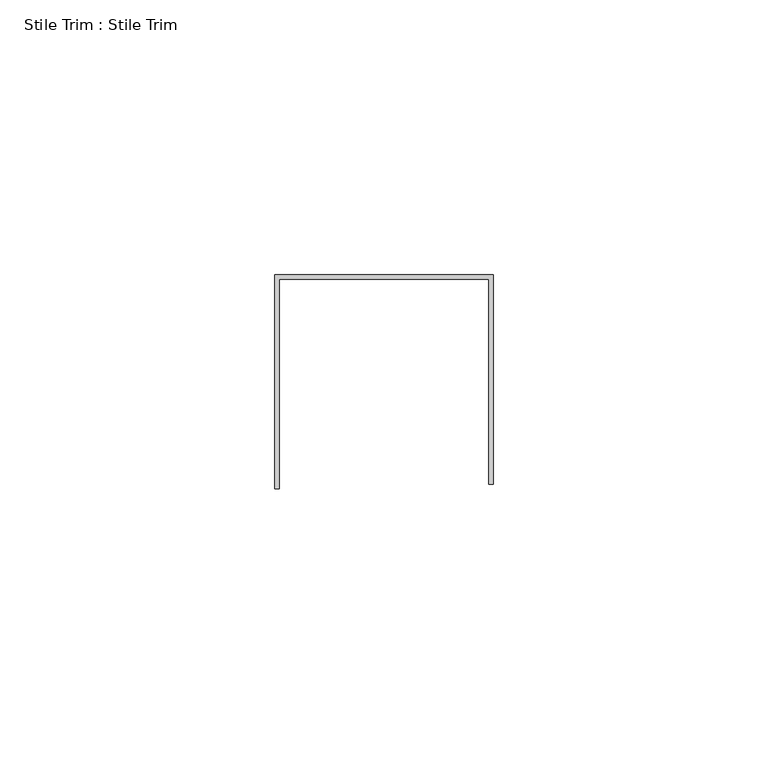
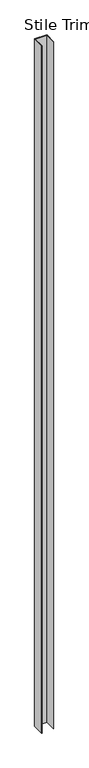
"""IFC4 building model written with IfcOpenShell, lengths in millimetres: proxy geometry, Stile Trim : Stile Trim."""

import ifcopenshell
import ifcopenshell.guid

model = None  # the IFC model being written
_history = None  # IfcOwnerHistory: only IFC2X3 demands one
_inside = {}  # id of a spatial element -> (the spatial element, [elements in it])
_under = {}  # id of a project, library or spatial element -> (it, [spatial elements below it])
_declared = {}  # id of a project -> (the project, [libraries it declares])
_typed = {}  # id of a type object -> (the type object, [elements of that type])
_made_of = {}  # id of a material, layer set ... -> (it, [elements and type objects made of it])


def new_model(schema):
    """Start an empty IFC model of exactly this schema.

    Asked for "IFC4X3", IfcOpenShell would pick the latest addendum, in which some entities
    have other attributes; the version numbers below select the first issue.
    IFC2X3 requires an IfcOwnerHistory on every rooted entity: one is made here for all.
    """
    global model, _history
    if schema == "IFC4X3":
        model = ifcopenshell.file(schema_version=(4, 3, 0, 0))
    else:
        model = ifcopenshell.file(schema=schema)
    _inside.clear()
    _under.clear()
    _declared.clear()
    _typed.clear()
    _made_of.clear()
    _history = None
    if model.schema == "IFC2X3":
        org = make("IfcOrganization", Name="unknown")
        user = make(
            "IfcPersonAndOrganization",
            ThePerson=make("IfcPerson", FamilyName="unknown"),
            TheOrganization=org,
        )
        app = make(
            "IfcApplication",
            ApplicationDeveloper=org,
            Version="unknown",
            ApplicationFullName="unknown",
            ApplicationIdentifier="unknown",
        )
        _history = make(
            "IfcOwnerHistory",
            OwningUser=user,
            OwningApplication=app,
            ChangeAction="ADDED",
            CreationDate=0,
        )
    return model


def make(cls, **values):
    """One entity of the class cls with the attributes given. An attribute that is None is left unset."""
    return model.create_entity(
        cls, **{name: value for name, value in values.items() if value is not None}
    )


def rooted(cls, **values):
    """An entity with a GlobalId (a new one), such as an element, a storey or a relation."""
    return make(cls, GlobalId=ifcopenshell.guid.new(), OwnerHistory=_history, **values)


def si_unit(unit_type, name, prefix=None):
    """IfcSIUnit, for example si_unit("LENGTHUNIT", "METRE", prefix="MILLI")."""
    return make("IfcSIUnit", UnitType=unit_type, Prefix=prefix, Name=name)


def assignment(units):
    """IfcUnitAssignment: the units of a project."""
    return None if units is None else make("IfcUnitAssignment", Units=units)


def point(xyz):
    """IfcCartesianPoint."""
    return None if xyz is None else make("IfcCartesianPoint", Coordinates=xyz)


def direction(xyz):
    """IfcDirection."""
    return None if xyz is None else make("IfcDirection", DirectionRatios=xyz)


def frame(location, z_axis=None, x_axis=None):
    """IfcAxis2Placement3D, a coordinate frame: its origin and axes. An axis left out is left unset."""
    return make(
        "IfcAxis2Placement3D",
        Location=point(location),
        Axis=direction(z_axis),
        RefDirection=direction(x_axis),
    )


def origin():
    """The frame at (0, 0, 0) with its axes left unset."""
    return frame((0.0, 0.0, 0.0))


def place(relative_to, where):
    """IfcLocalPlacement: puts the frame where relative to a parent placement (None: the world)."""
    return make(
        "IfcLocalPlacement", PlacementRelTo=relative_to, RelativePlacement=where
    )


def context(
    kind, dimensions, precision=None, world=None, true_north=None, identifier=None
):
    """IfcGeometricRepresentationContext, for example the 3D "Model" context."""
    return make(
        "IfcGeometricRepresentationContext",
        ContextIdentifier=identifier,
        ContextType=kind,
        CoordinateSpaceDimension=dimensions,
        Precision=precision,
        WorldCoordinateSystem=world,
        TrueNorth=true_north,
    )


def project(units=None, contexts=None):
    """IfcProject with its units and contexts."""
    return rooted(
        "IfcProject",
        Name="project",
        RepresentationContexts=contexts,
        UnitsInContext=assignment(units),
    )


def spatial(cls, under=None, at=None, **own):
    """A site, building, storey or space (cls), placed at a placement, below another one or the project."""
    s = rooted(cls, ObjectPlacement=at, **own)
    if under is not None:
        _under.setdefault(under.id(), (under, []))[1].append(s)
    return s


def polyline(points):
    """IfcPolyline through the points."""
    return make("IfcPolyline", Points=[point(p) for p in points])


def outline(outer, holes=None, kind="AREA"):
    """IfcArbitraryClosedProfileDef: a profile drawn as a closed curve; with holes, ...WithVoids."""
    if holes is None:
        return make("IfcArbitraryClosedProfileDef", ProfileType=kind, OuterCurve=outer)
    return make(
        "IfcArbitraryProfileDefWithVoids",
        ProfileType=kind,
        OuterCurve=outer,
        InnerCurves=holes,
    )


def extrude(swept, where, along, depth):
    """IfcExtrudedAreaSolid: the profile swept, set in the frame where, extruded along a direction by depth."""
    return make(
        "IfcExtrudedAreaSolid",
        SweptArea=swept,
        Position=where,
        ExtrudedDirection=direction(along),
        Depth=depth,
    )


def shape(context_of_items, identifier, shape_type, items):
    """IfcShapeRepresentation: the items that make up one representation, for example the "Body"."""
    return make(
        "IfcShapeRepresentation",
        ContextOfItems=context_of_items,
        RepresentationIdentifier=identifier,
        RepresentationType=shape_type,
        Items=items,
    )


def source(mapping_origin, context_of_items, identifier, shape_type, items):
    """IfcRepresentationMap: a shape defined once, which mapped items show again and again."""
    return make(
        "IfcRepresentationMap",
        MappingOrigin=mapping_origin,
        MappedRepresentation=shape(context_of_items, identifier, shape_type, items),
    )


def transform(
    local_origin,
    x_axis=None,
    y_axis=None,
    z_axis=None,
    scale=None,
    scale2=None,
    scale3=None,
    uniform=True,
):
    """IfcCartesianTransformationOperator3D, or its non-uniform kind. x_axis, y_axis, z_axis: its Axis1, 2, 3."""
    if uniform:
        return make(
            "IfcCartesianTransformationOperator3D",
            Axis1=direction(x_axis),
            Axis2=direction(y_axis),
            LocalOrigin=point(local_origin),
            Scale=scale,
            Axis3=direction(z_axis),
        )
    return make(
        "IfcCartesianTransformationOperator3DnonUniform",
        Axis1=direction(x_axis),
        Axis2=direction(y_axis),
        LocalOrigin=point(local_origin),
        Scale=scale,
        Axis3=direction(z_axis),
        Scale2=scale2,
        Scale3=scale3,
    )


def mapped(mapping_source, mapping_target):
    """IfcMappedItem: shows the shape of a source again, moved by a transform."""
    return make(
        "IfcMappedItem", MappingSource=mapping_source, MappingTarget=mapping_target
    )


def made_of(thing, what):
    """Note that an element or type object is made of a material, layer set ...; save() writes the relation."""
    if what is not None:
        _made_of.setdefault(what.id(), (what, []))[1].append(thing)
    return thing


def element(
    cls,
    number,
    at=None,
    inside=None,
    cuts=None,
    type_object=None,
    material=None,
    context=None,
    identifier="Body",
    shape_type=None,
    held_by="IfcProductDefinitionShape",
    body=None,
    shapes=None,
    **own,
):
    """One element of the class cls, such as IfcWall. Its Tag is "e" and its number.

    at: its placement. inside: the storey or other place that contains it. cuts: it is an
    opening in that element (IfcRelVoidsElement). A single representation is given by context,
    identifier, shape_type and body (its items); several are given by shapes. held_by: the class
    of the entity that holds the representations. save() writes the other relations.
    """
    e = rooted(cls, Tag="e%d" % number, ObjectPlacement=at, **own)
    if body is not None:
        shapes = [shape(context, identifier, shape_type, body)]
    if shapes is not None:
        e.Representation = make(held_by, Representations=shapes)
    if inside is not None:
        _inside.setdefault(inside.id(), (inside, []))[1].append(e)
    if cuts is not None:
        rooted(
            "IfcRelVoidsElement", RelatingBuildingElement=cuts, RelatedOpeningElement=e
        )
    if type_object is not None:
        _typed.setdefault(type_object.id(), (type_object, []))[1].append(e)
    return made_of(e, material)


def aggregate(whole, parts):
    """IfcRelAggregates: a whole, such as a stair, and the parts it consists of."""
    return rooted("IfcRelAggregates", RelatingObject=whole, RelatedObjects=parts)


def save(model, path):
    """Write the relations noted so far, then the file.

    IfcRelAggregates (storeys below a building ...), IfcRelContainedInSpatialStructure (elements
    in a storey), IfcRelDefinesByType, IfcRelAssociatesMaterial and IfcRelDeclares: one each for
    every whole, place, type object, material and project.
    """
    for whole, parts in _under.values():
        aggregate(whole, parts)
    for where, things in _inside.values():
        rooted(
            "IfcRelContainedInSpatialStructure",
            RelatedElements=things,
            RelatingStructure=where,
        )
    for kind, things in _typed.values():
        rooted("IfcRelDefinesByType", RelatedObjects=things, RelatingType=kind)
    for what, things in _made_of.values():
        rooted("IfcRelAssociatesMaterial", RelatedObjects=things, RelatingMaterial=what)
    for by, libraries in _declared.values():
        rooted("IfcRelDeclares", RelatingContext=by, RelatedDefinitions=libraries)
    model.write(path)


def stile_trim_stile_trim_02668cd7(model_context):
    return source(origin(), model_context, "Body", "SweptSolid", [
        extrude(outline(polyline([(587327.0060739, -531784.4789841), (587366.6808739, -531784.4789841), (587366.6808739, -531822.5789841), (587365.8934739, -531822.5789841), (587365.8934739, -531785.2663841), (587327.7934739, -531785.2663841), (587327.7934739, -531823.3663841), (587327.0060739, -531823.3663841), (587327.0060739, -531784.4789841)])), frame((0.0, 0.0, 50.8), z_axis=(0.0, 0.0, 1.0), x_axis=(1.0, 0.0, 0.0)), (0.0, 0.0, 1.0), 2350.3929688),
    ])


if __name__ == "__main__":
    model = new_model("IFC4")
    model_context = context("Model", 3, world=origin())
    ifc_project = project(units=[si_unit("LENGTHUNIT", "METRE", prefix="MILLI")], contexts=[model_context])
    site = spatial("IfcSite", under=ifc_project)
    building = spatial("IfcBuilding", under=site)
    placement = place(None, origin())
    stile_trim_stile_trim_shape = stile_trim_stile_trim_02668cd7(model_context)
    element("IfcBuildingElementProxy", 1, Name="Stile Trim : Stile Trim", ObjectType="Stile Trim : Stile Trim", at=placement, inside=building, context=model_context, shape_type="MappedRepresentation", body=[
        mapped(stile_trim_stile_trim_shape, transform((0.0, 0.0, 0.0), x_axis=(1.0, 0.0, 0.0), y_axis=(0.0, 1.0, 0.0), z_axis=(0.0, 0.0, 1.0))),
    ])
    save(model, "model.ifc")

# Revit data of these elements
# Element 1 (IfcBuildingElementProxy, "Stile Trim : Stile Trim")
#   Materials on its faces: "EDGE TRIM BY MTL PANEL MFR."
# Materials
#   "EDGE TRIM BY MTL PANEL MFR.": class "Generic", colour RGB 239 242 240, transparency 0, Cost = 0
